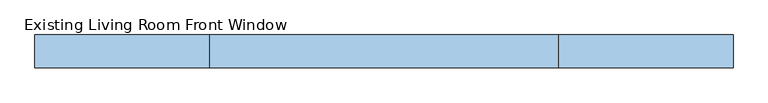
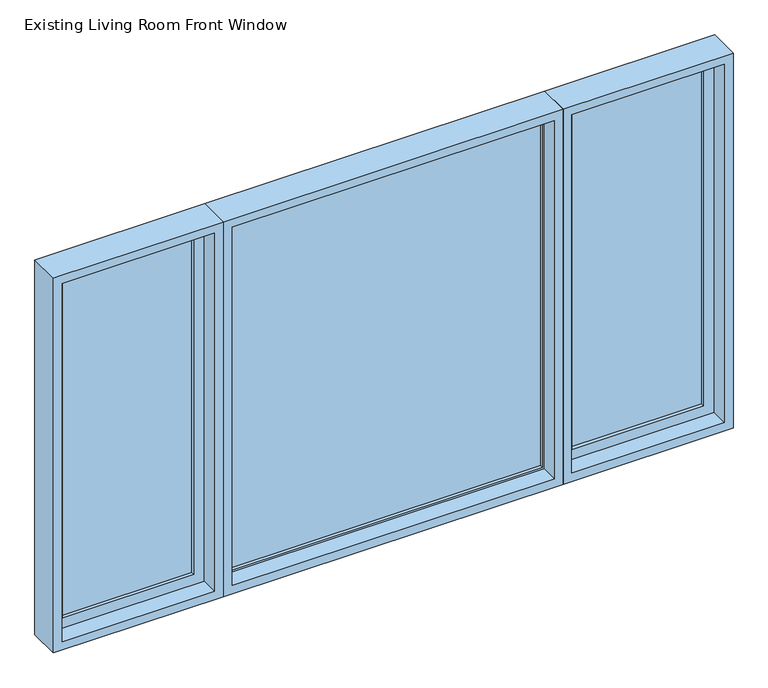
"""IFC4 building model written with IfcOpenShell, lengths in millimetres: window geometry, Existing Living Room Front Window."""

from ifc_helpers import new_model, si_unit, frame, origin, place, context, project, spatial, polyline, outline, extrude, faceted_brep, source, transform, mapped, element, save


def existing_living_room_front_window_917c3268(model_context):
    return source(origin(), model_context, "Body", "SolidModel", [
        extrude(outline(polyline([(-1149.35, 158.75), (-679.45, 158.75), (-679.45, 152.4), (-1149.35, 152.4), (-1149.35, 158.75)])), frame((0.0, 0.0, 984.25), z_axis=(0.0, 0.0, 1.0), x_axis=(1.0, 0.0, 0.0)), (0.0, 0.0, 1.0), 1282.7),
        extrude(outline(polyline([(-679.45, 139.7), (-1149.35, 139.7), (-1149.35, 146.05), (-679.45, 146.05), (-679.45, 139.7)])), frame((0.0, 0.0, 984.25), z_axis=(0.0, 0.0, 1.0), x_axis=(1.0, 0.0, 0.0)), (0.0, 0.0, 1.0), 1282.7),
        extrude(outline(polyline([(2324.1, -622.3), (2324.1, -1206.5), (927.1, -1206.5), (927.1, -622.3), (2324.1, -622.3)]), holes=[polyline([(2266.95, -1149.35), (2266.95, -679.45), (984.25, -679.45), (984.25, -1149.35), (2266.95, -1149.35)])]), frame((0.0, 127.0, 0.0), z_axis=(0.0, 1.0, 0.0), x_axis=(0.0, 0.0, 1.0)), (0.0, 0.0, 1.0), 44.45),
        faceted_brep([(-1187.45, 127.0, 2305.05), (-641.35, 127.0, 2305.05), (-641.35, 63.5, 2305.05), (-1187.45, 63.5, 2305.05), (-1206.5, 177.8, 2324.1), (-622.3, 177.8, 2324.1), (-622.3, 127.0, 2324.1), (-1206.5, 127.0, 2324.1), (-1219.2, 63.5, 2336.8), (-609.6, 63.5, 2336.8), (-609.6, 177.8, 2336.8), (-1219.2, 177.8, 2336.8), (-641.35, 127.0, 946.15), (-641.35, 63.5, 946.15), (-622.3, 177.8, 927.1), (-622.3, 127.0, 927.1), (-609.6, 63.5, 914.4), (-609.6, 177.8, 914.4), (-1187.45, 127.0, 946.15), (-1187.45, 63.5, 946.15), (-1206.5, 177.8, 927.1), (-1206.5, 127.0, 927.1), (-1219.2, 63.5, 914.4), (-1219.2, 177.8, 914.4)], [[[0, 1, 2, 3]], [[4, 5, 6, 7]], [[8, 9, 10, 11]], [[1, 12, 13, 2]], [[5, 14, 15, 6]], [[9, 16, 17, 10]], [[12, 18, 19, 13]], [[14, 20, 21, 15]], [[16, 22, 23, 17]], [[9, 8, 22, 16], [3, 2, 13, 19]], [[18, 0, 3, 19]], [[7, 6, 15, 21], [1, 0, 18, 12]], [[20, 4, 7, 21]], [[22, 8, 11, 23]], [[11, 10, 17, 23], [5, 4, 20, 14]]]),
        extrude(outline(polyline([(679.45, 158.75), (1149.35, 158.75), (1149.35, 152.4), (679.45, 152.4), (679.45, 158.75)])), frame((0.0, 0.0, 984.25), z_axis=(0.0, 0.0, 1.0), x_axis=(1.0, 0.0, 0.0)), (0.0, 0.0, 1.0), 1282.7),
        extrude(outline(polyline([(1149.35, 139.7), (679.45, 139.7), (679.45, 146.05), (1149.35, 146.05), (1149.35, 139.7)])), frame((0.0, 0.0, 984.25), z_axis=(0.0, 0.0, 1.0), x_axis=(1.0, 0.0, 0.0)), (0.0, 0.0, 1.0), 1282.7),
        extrude(outline(polyline([(2324.1, 1206.5), (2324.1, 622.3), (927.1, 622.3), (927.1, 1206.5), (2324.1, 1206.5)]), holes=[polyline([(2266.95, 679.45), (2266.95, 1149.35), (984.25, 1149.35), (984.25, 679.45), (2266.95, 679.45)])]), frame((0.0, 127.0, 0.0), z_axis=(0.0, 1.0, 0.0), x_axis=(0.0, 0.0, 1.0)), (0.0, 0.0, 1.0), 44.45),
        faceted_brep([(641.35, 127.0, 2305.05), (1187.45, 127.0, 2305.05), (1187.45, 63.5, 2305.05), (641.35, 63.5, 2305.05), (622.3, 177.8, 2324.1), (1206.5, 177.8, 2324.1), (1206.5, 127.0, 2324.1), (622.3, 127.0, 2324.1), (609.6, 63.5, 2336.8), (1219.2, 63.5, 2336.8), (1219.2, 177.8, 2336.8), (609.6, 177.8, 2336.8), (1187.45, 127.0, 946.15), (1187.45, 63.5, 946.15), (1206.5, 177.8, 927.1), (1206.5, 127.0, 927.1), (1219.2, 63.5, 914.4), (1219.2, 177.8, 914.4), (641.35, 127.0, 946.15), (641.35, 63.5, 946.15), (622.3, 177.8, 927.1), (622.3, 127.0, 927.1), (609.6, 63.5, 914.4), (609.6, 177.8, 914.4)], [[[0, 1, 2, 3]], [[4, 5, 6, 7]], [[8, 9, 10, 11]], [[1, 12, 13, 2]], [[5, 14, 15, 6]], [[9, 16, 17, 10]], [[12, 18, 19, 13]], [[14, 20, 21, 15]], [[16, 22, 23, 17]], [[9, 8, 22, 16], [3, 2, 13, 19]], [[18, 0, 3, 19]], [[7, 6, 15, 21], [1, 0, 18, 12]], [[20, 4, 7, 21]], [[22, 8, 11, 23]], [[11, 10, 17, 23], [5, 4, 20, 14]]]),
        extrude(outline(polyline([(-571.5, 158.75), (571.5, 158.75), (571.5, 152.4), (-571.5, 152.4), (-571.5, 158.75)])), frame((0.0, 0.0, 952.5), z_axis=(0.0, 0.0, 1.0), x_axis=(1.0, 0.0, 0.0)), (0.0, 0.0, 1.0), 1346.2),
        extrude(outline(polyline([(571.5, 139.7), (-571.5, 139.7), (-571.5, 146.05), (571.5, 146.05), (571.5, 139.7)])), frame((0.0, 0.0, 952.5), z_axis=(0.0, 0.0, 1.0), x_axis=(1.0, 0.0, 0.0)), (0.0, 0.0, 1.0), 1346.2),
        extrude(outline(polyline([(927.1, -596.9), (927.1, 596.9), (2324.1, 596.9), (2324.1, -596.9), (927.1, -596.9)]), holes=[polyline([(952.5, 571.5), (952.5, -571.5), (2298.7, -571.5), (2298.7, 571.5), (952.5, 571.5)])]), frame((0.0, 127.0, 0.0), z_axis=(0.0, 1.0, 0.0), x_axis=(0.0, 0.0, 1.0)), (0.0, 0.0, 1.0), 44.45),
        faceted_brep([(-609.6, 63.5, 2336.8), (609.6, 63.5, 2336.8), (609.6, 177.8, 2336.8), (-609.6, 177.8, 2336.8), (609.6, 63.5, 914.4), (609.6, 177.8, 914.4), (-609.6, 63.5, 914.4), (-609.6, 177.8, 914.4), (-577.85, 63.5, 2305.05), (577.85, 63.5, 2305.05), (577.85, 63.5, 946.15), (-577.85, 63.5, 946.15), (596.9, 177.8, 2324.1), (-596.9, 177.8, 2324.1), (-596.9, 177.8, 927.1), (596.9, 177.8, 927.1), (-577.85, 127.0, 2305.05), (577.85, 127.0, 2305.05), (596.9, 127.0, 2324.1), (-596.9, 127.0, 2324.1), (577.85, 127.0, 946.15), (596.9, 127.0, 927.1), (-577.85, 127.0, 946.15), (-596.9, 127.0, 927.1)], [[[0, 1, 2, 3]], [[1, 4, 5, 2]], [[4, 6, 7, 5]], [[1, 0, 6, 4], [8, 9, 10, 11]], [[6, 0, 3, 7]], [[3, 2, 5, 7], [12, 13, 14, 15]], [[16, 17, 9, 8]], [[13, 12, 18, 19]], [[17, 20, 10, 9]], [[12, 15, 21, 18]], [[20, 22, 11, 10]], [[15, 14, 23, 21]], [[22, 16, 8, 11]], [[19, 18, 21, 23], [17, 16, 22, 20]], [[14, 13, 19, 23]]]),
    ])


if __name__ == "__main__":
    model = new_model("IFC4")
    model_context = context("Model", 3, world=origin())
    ifc_project = project(units=[si_unit("LENGTHUNIT", "METRE", prefix="MILLI")], contexts=[model_context])
    site = spatial("IfcSite", under=ifc_project)
    building = spatial("IfcBuilding", under=site)
    placement = place(None, origin())
    existing_living_room_front_window_shape = existing_living_room_front_window_917c3268(model_context)
    element("IfcWindow", 1, ObjectType="Existing Living Room Front Window : (2) 2'-0\" x 4'-8\" CS + 4'-0\" x 4'-8\" FX", at=placement, inside=building, context=model_context, shape_type="MappedRepresentation", body=[
        mapped(existing_living_room_front_window_shape, transform((0.0, 0.0, 0.0), x_axis=(1.0, 0.0, 0.0), y_axis=(0.0, 1.0, 0.0), z_axis=(0.0, 0.0, 1.0))),
    ])
    save(model, "model.ifc")

# Revit data of these elements
# Type "Existing Living Room Front Window : (2) 2'-0\" x 4'-8\" CS + 4'-0\" x 4'-8\" FX"
#   Type Mark = "31"
#   Analytic Construction = "<None>"
#   Window Inset = 0' - 0 3/4"
#   Side Window Width = 2' - 0"
#   Side Window Location = 2' - 0"
#   Middle Window Width = 4' - 0"
#   Height = 4' - 8"
#   Default Sill Height = 3' - 0"
#   Width = 8' - 0"
#   Top Muntin Visibility = yes
#   Side Window Nested Trim Visibility = no
#   Interior Trim Visibility [instance default] = yes
#   Fixed Muntin Visibility = no
#   Exterior Trim Visibility [instance default] = yes
#   Define Thermal Properties by = 1
#   Bottom Muntin Visibility = yes
#   Sash Material = Clad - White
#   Right Side Window Type = element 472099
#   Left Side Window Type = element 472100
#   Interior Trim = Trim-Window-Interior-Flat : Picture Frame
#   Interior Trim Material = Maple - Semigloss(Rotated)
#   Interior Frame Material = Maple - Semigloss(Rotated)
#   Glass Pane Material = Glass, Clear Glazing
#   Exterior Trim Material = Clad - White
#   Exterior Trim = Trim-Window-Exterior-Flat : with Sill
#   Exterior Frame Material = Clad - White
#   Rough Width = 0
#   Rough Height = 0
#   Wall Closure = (empty or 0)
# Element 1 (IfcWindow, "Existing Living Room Front Window : (2) 2'-0\" x 4'-8\" CS + 4'-0\" x 4'-8\" FX")
#   Materials on its faces: "Maple - Semigloss(Rotated)", "Glass", "Clad - White", "Glass, Clear Glazing"
# Materials
#   "Clad - White": class "Wood", colour RGB 245 245 243, transparency 0, Cost = 0
#   "Maple - Semigloss(Rotated)": class "Wood", colour RGB 196 161 118, transparency 0, Description = "Acer Saccharum", Cost = 0
#   "Glass, Clear Glazing": class "Glass", colour RGB 245 245 243, transparency 1, Description = "Clear glazing", Cost = 0
#   "Glass": class "Glass", colour RGB 0 128 192, transparency 0.75, Description = "Soda Lime Glass", Cost = 0
